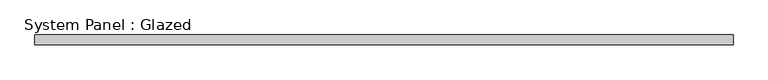
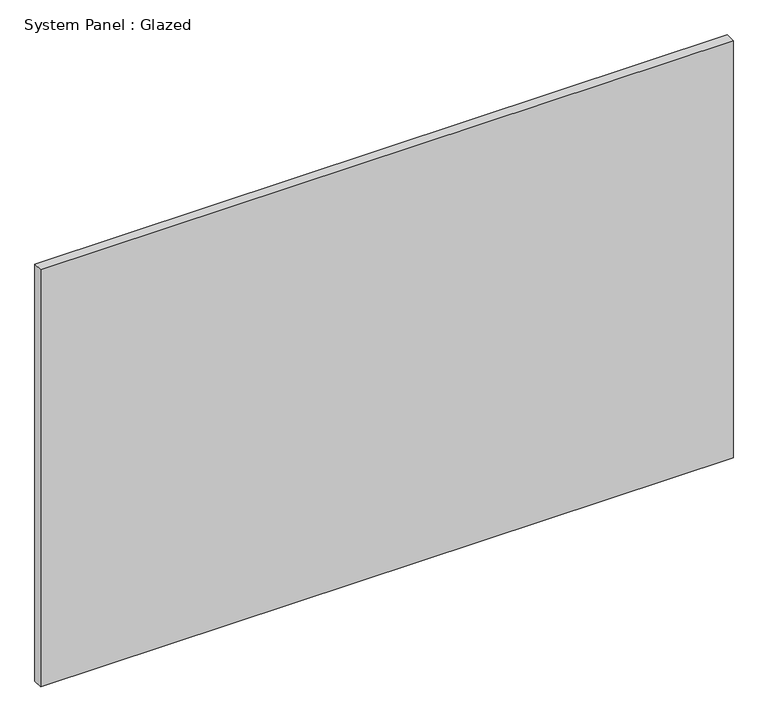
"""IFC4 building model written with IfcOpenShell, lengths in millimetres: plate geometry, System Panel : Glazed."""

from ifc_helpers import new_model, si_unit, origin, origin_with_axes, place, context, project, spatial, polyline, outline, extrude, source, transform, mapped, element, save


def system_panel_glazed_d529eb93(model_context):
    return source(origin(), model_context, "Body", "SweptSolid", [
        extrude(outline(polyline([(882.65, -44.45), (-882.65, -44.45), (-882.65, -19.05), (882.65, -19.05), (882.65, -44.45)])), origin_with_axes(), (0.0, 0.0, 1.0), 1123.95),
    ])


if __name__ == "__main__":
    model = new_model("IFC4")
    model_context = context("Model", 3, world=origin())
    ifc_project = project(units=[si_unit("LENGTHUNIT", "METRE", prefix="MILLI")], contexts=[model_context])
    site = spatial("IfcSite", under=ifc_project)
    building = spatial("IfcBuilding", under=site)
    placement = place(None, origin())
    system_panel_glazed_shape = system_panel_glazed_d529eb93(model_context)
    element("IfcPlate", 1, ObjectType="System Panel : Glazed", at=placement, inside=building, context=model_context, shape_type="MappedRepresentation", body=[
        mapped(system_panel_glazed_shape, transform((0.0, 0.0, 0.0), x_axis=(1.0, 0.0, 0.0), y_axis=(0.0, 1.0, 0.0), z_axis=(0.0, 0.0, 1.0))),
    ])
    save(model, "model.ifc")

# Revit data of these elements
# Type "System Panel : Glazed"
#   Construction Type Id = "GSP4R"
#   Analytic Construction = "1/8 in Pilkington single glazing"
#   Visual Light Transmittance = 0.9
#   Solar Heat Gain Coefficient = 0.86
#   Heat Transfer Coefficient (U) = 1.18115 BTU/(h·ft²·°F)
#   Define Thermal Properties by = 1
# Element 1 (IfcPlate, "System Panel : Glazed")
#   Materials on its faces: "Glass"
# Materials
#   "Glass": class "Glass", colour RGB 0 128 192, transparency 0.75, Description = "Soda Lime Glass", Cost = 0
